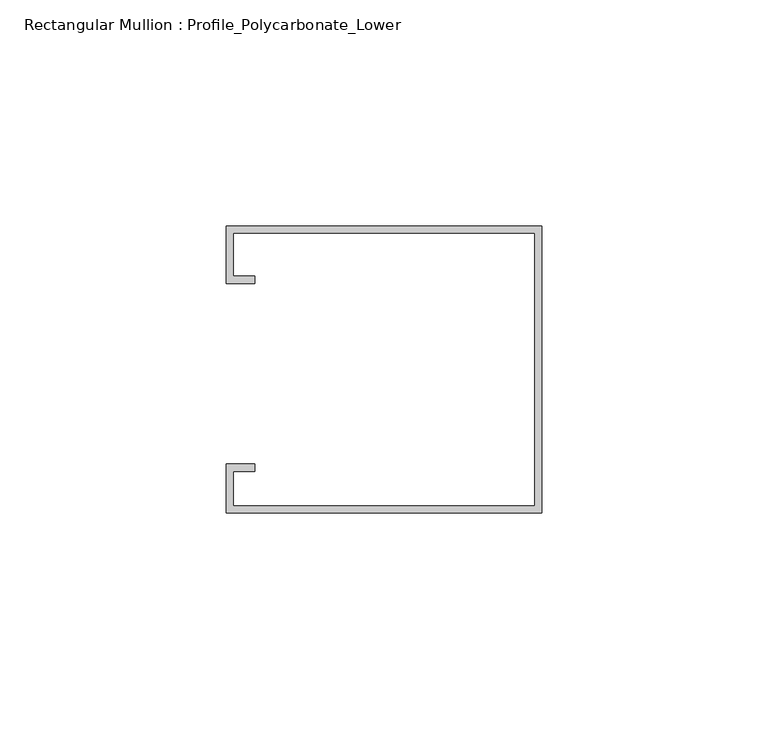
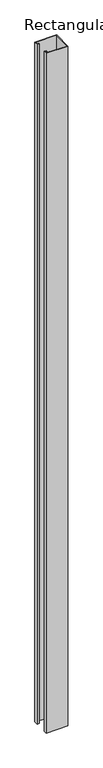
"""IFC4 building model written with IfcOpenShell, lengths in millimetres: member geometry, Rectangular Mullion : Profile_Polycarbonate_Lower."""

from ifc_helpers import new_model, si_unit, frame, origin, place, context, project, spatial, polyline, outline, extrude, source, transform, mapped, element, save


def rectangular_mullion_profile_polycarbonate_lower_3a4ba5bc(model_context):
    return source(origin(), model_context, "Body", "SweptSolid", [
        extrude(outline(polyline([(0.0, 32.7), (0.0, -30.8), (-69.85, -30.8), (-69.85, -20.0), (-63.5, -20.0), (-63.5, -21.5875), (-68.2625, -21.5875), (-68.2625, -29.2125), (-1.5875, -29.2125), (-1.5875, 31.1125), (-68.2625, 31.1125), (-68.2625, 21.5875), (-63.5, 21.5875), (-63.5, 20.0), (-69.85, 20.0), (-69.85, 32.7), (0.0, 32.7)])), frame((0.0, 0.0, -2317.75), z_axis=(0.0, 0.0, 1.0), x_axis=(1.0, 0.0, 0.0)), (0.0, 0.0, 1.0), 2317.75),
    ])


if __name__ == "__main__":
    model = new_model("IFC4")
    model_context = context("Model", 3, world=origin())
    ifc_project = project(units=[si_unit("LENGTHUNIT", "METRE", prefix="MILLI")], contexts=[model_context])
    site = spatial("IfcSite", under=ifc_project)
    building = spatial("IfcBuilding", under=site)
    placement = place(None, origin())
    rectangular_mullion_profile_polycarbonate_lower_shape = rectangular_mullion_profile_polycarbonate_lower_3a4ba5bc(model_context)
    element("IfcMember", 1, ObjectType="Rectangular Mullion : Profile_Polycarbonate_Lower", at=placement, inside=building, context=model_context, shape_type="MappedRepresentation", body=[
        mapped(rectangular_mullion_profile_polycarbonate_lower_shape, transform((0.0, 0.0, 0.0), x_axis=(1.0, 0.0, 0.0), y_axis=(0.0, 1.0, 0.0), z_axis=(0.0, 0.0, 1.0))),
    ])
    save(model, "model.ifc")

# Revit data of these elements
# Type "Rectangular Mullion : Profile_Polycarbonate_Lower"
#   built-in parameter 1007322 = 0.208333 (stored number, unit not read)
#   built-in parameter 1007321 = 0 (stored number, unit not read)
#   built-in parameter 1007320 = 0.00520833 (stored number, unit not read)
